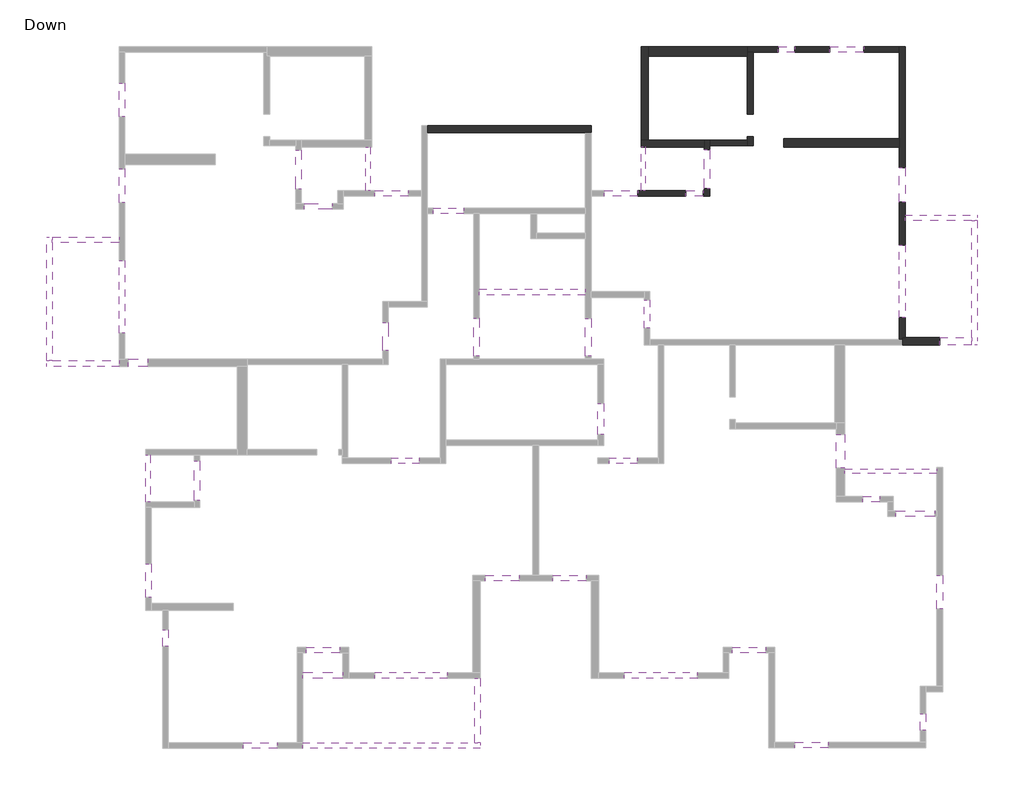
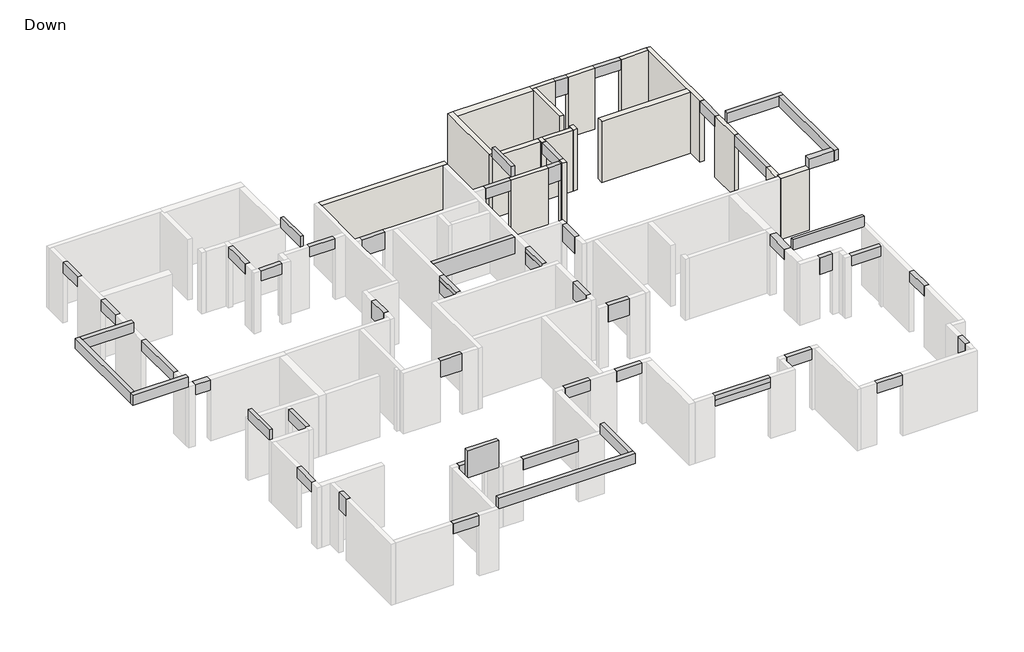
# One storey, part 3 of 3: 52 beams, 19 walls.
# Revit data of these elements (continued)
# Element 38 (IfcBeam, "Concrete Rectengular Beam : 20/82") (continued)
#   Phase Created = New Construction
#   Materials on its faces: "Concrete"
# Element 39 (IfcBeam, "Concrete Rectengular Beam : 20/82")
#   Comments = ""
#   Mark = "B42"
#   SOFiSTiK_AMG_Comments = ""
#   SOFiSTiK_AMG_Scheduled = yes
#   SOFiSTiK_AMG_Adjusted = yes
#   Structural Material = Concrete
#   Phase Created = New Construction
#   Materials on its faces: "Concrete"
# Element 40 (IfcBeam, "Concrete Rectengular Beam : 20/82")
#   Comments = ""
#   Mark = "B43"
#   SOFiSTiK_AMG_Comments = ""
#   SOFiSTiK_AMG_Scheduled = yes
#   SOFiSTiK_AMG_Adjusted = yes
#   Structural Material = Concrete
#   Phase Created = New Construction
#   Materials on its faces: "Concrete"
# Element 41 (IfcBeam, "Concrete Rectengular Beam : 20/82")
#   Comments = ""
#   Mark = "B44"
#   SOFiSTiK_AMG_Comments = ""
#   SOFiSTiK_AMG_Scheduled = yes
#   SOFiSTiK_AMG_Adjusted = yes
#   Structural Material = Concrete
#   Phase Created = New Construction
#   Materials on its faces: "Concrete"
# Element 42 (IfcBeam, "Concrete Rectengular Beam : 20/82")
#   Comments = ""
#   Mark = "B45"
#   SOFiSTiK_AMG_Comments = ""
#   SOFiSTiK_AMG_Scheduled = yes
#   SOFiSTiK_AMG_Adjusted = yes
#   Structural Material = Concrete
#   Phase Created = New Construction
#   Materials on its faces: "Concrete"
# Element 43 (IfcBeam, "Concrete Rectengular Beam : 20/82")
#   Comments = ""
#   Mark = "B46"
#   SOFiSTiK_AMG_Comments = ""
#   SOFiSTiK_AMG_Scheduled = yes
#   SOFiSTiK_AMG_Adjusted = yes
#   Structural Material = Concrete
#   Phase Created = New Construction
#   Materials on its faces: "Concrete"
# Element 44 (IfcBeam, "Concrete Rectengular Beam : 20/82")
#   Comments = ""
#   Mark = "B47"
#   SOFiSTiK_AMG_Comments = ""
#   SOFiSTiK_AMG_Scheduled = yes
#   SOFiSTiK_AMG_Adjusted = yes
#   Structural Material = Concrete
#   Phase Created = New Construction
#   Materials on its faces: "Concrete"
# Element 45 (IfcBeam, "Concrete Rectengular Beam : 20/82")
#   Comments = ""
#   Mark = "B48"
#   SOFiSTiK_AMG_Comments = ""
#   SOFiSTiK_AMG_Scheduled = yes
#   SOFiSTiK_AMG_Adjusted = yes
#   Structural Material = Concrete
#   Phase Created = New Construction
#   Materials on its faces: "Concrete"
# Element 46 (IfcBeam, "Concrete Rectengular Beam : 20/82")
#   Comments = ""
#   Mark = "B49"
#   SOFiSTiK_AMG_Comments = ""
#   SOFiSTiK_AMG_Scheduled = yes
#   SOFiSTiK_AMG_Adjusted = yes
#   Structural Material = Concrete
#   Phase Created = New Construction
#   Materials on its faces: "Concrete"
# Element 47 (IfcBeam, "Concrete Rectengular Beam : 20/82")
#   Comments = ""
#   Mark = "B50"
#   SOFiSTiK_AMG_Comments = ""
#   SOFiSTiK_AMG_Scheduled = yes
#   SOFiSTiK_AMG_Adjusted = yes
#   Structural Material = Concrete
#   Phase Created = New Construction
#   Materials on its faces: "Concrete"
# Element 48 (IfcBeam, "Concrete Rectengular Beam : 20/82")
#   Comments = ""
#   Mark = "B51"
#   SOFiSTiK_AMG_Comments = ""
#   SOFiSTiK_AMG_Scheduled = yes
#   SOFiSTiK_AMG_Adjusted = yes
#   Structural Material = Concrete
#   Phase Created = New Construction
#   Materials on its faces: "Concrete"
# Element 49 (IfcBeam, "Concrete Rectengular Beam : 20/82")
#   Comments = ""
#   Mark = "B52"
#   SOFiSTiK_AMG_Comments = ""
#   SOFiSTiK_AMG_Scheduled = yes
#   SOFiSTiK_AMG_Adjusted = yes
#   Structural Material = Concrete
#   Phase Created = New Construction
#   Materials on its faces: "Concrete"
# Element 50 (IfcBeam, "Concrete Rectengular Beam : 27/50")
#   Comments = ""
#   Mark = "B53"
#   SOFiSTiK_AMG_Comments = ""
#   SOFiSTiK_AMG_Scheduled = yes
#   SOFiSTiK_AMG_Adjusted = yes
#   Structural Material = Concrete
#   Phase Created = New Construction
#   Materials on its faces: "Concrete"
# Element 51 (IfcBeam, "Concrete Rectengular Beam : 27/50")
#   Comments = ""
#   Mark = "B54"
#   SOFiSTiK_AMG_Comments = ""
#   SOFiSTiK_AMG_Scheduled = yes
#   SOFiSTiK_AMG_Adjusted = yes
#   Structural Material = Concrete
#   Phase Created = New Construction
#   Materials on its faces: "Concrete"
# Element 52 (IfcBeam, "Concrete Rectengular Beam : 30/50")
#   Comments = ""
#   Mark = "B55"
#   SOFiSTiK_AMG_Comments = ""
#   SOFiSTiK_AMG_Scheduled = yes
#   SOFiSTiK_AMG_Adjusted = yes
#   Structural Material = Concrete
#   Phase Created = New Construction
#   Materials on its faces: "Concrete"
# Element 53 (IfcWall, "20")
#   Comments = ""
#   Mark = "W87"
#   SOFiSTiK_EdgeZones = "W87"
#   SOFiSTiK_AMG_Comments = ""
#   Top Offset = 0 cm
#   Base Offset = 0 cm
#   wall height = 300 cm
#   SOFiSTiK_AMG_Scheduled = yes
#   SOFiSTiK_AMG_Adjusted = yes
#   Phase Created = New Construction
#   Base Constraint = Down
#   Top Constraint = Typical Floor
#   Materials on its faces: "Concrete"
# Element 54 (IfcWall, "20")
#   Comments = ""
#   Mark = "W88"
#   SOFiSTiK_EdgeZones = "W88"
#   SOFiSTiK_AMG_Comments = ""
#   Top Offset = 0 cm
#   Base Offset = 0 cm
#   wall height = 300 cm
#   SOFiSTiK_AMG_Scheduled = yes
#   SOFiSTiK_AMG_Adjusted = yes
#   Phase Created = New Construction
#   Base Constraint = Down
#   Top Constraint = Typical Floor
#   Materials on its faces: "Concrete"
# Element 55 (IfcWall, "20")
#   Comments = ""
#   Mark = "W89"
#   SOFiSTiK_EdgeZones = "W89"
#   SOFiSTiK_AMG_Comments = ""
#   Top Offset = 0 cm
#   Base Offset = 0 cm
#   wall height = 300 cm
#   SOFiSTiK_AMG_Scheduled = yes
#   SOFiSTiK_AMG_Adjusted = yes
#   Phase Created = New Construction
#   Base Constraint = Down
#   Top Constraint = Typical Floor
#   Materials on its faces: "Concrete"
# Element 56 (IfcWall, "20")
#   Comments = ""
#   Mark = "W90"
#   SOFiSTiK_EdgeZones = "W90"
#   SOFiSTiK_AMG_Comments = ""
#   Top Offset = 0 cm
#   Base Offset = 0 cm
#   wall height = 300 cm
#   SOFiSTiK_AMG_Scheduled = yes
#   SOFiSTiK_AMG_Adjusted = yes
#   Phase Created = New Construction
#   Base Constraint = Down
#   Top Constraint = Typical Floor
#   Materials on its faces: "Concrete"
# Element 57 (IfcWall, "20")
#   Comments = ""
#   Mark = "W91"
#   SOFiSTiK_EdgeZones = "W91"
#   SOFiSTiK_AMG_Comments = ""
#   Top Offset = 0 cm
#   Base Offset = 0 cm
#   wall height = 300 cm
#   SOFiSTiK_AMG_Scheduled = yes
#   SOFiSTiK_AMG_Adjusted = yes
#   Phase Created = New Construction
#   Base Constraint = Down
#   Top Constraint = Typical Floor
#   Materials on its faces: "Concrete"
# Element 58 (IfcWall, "20")
#   Comments = ""
#   Mark = "W92"
#   SOFiSTiK_EdgeZones = "W92"
#   SOFiSTiK_AMG_Comments = ""
#   Top Offset = 0 cm
#   Base Offset = 0 cm
#   wall height = 300 cm
#   SOFiSTiK_AMG_Scheduled = yes
#   SOFiSTiK_AMG_Adjusted = yes
#   Phase Created = New Construction
#   Base Constraint = Down
#   Top Constraint = Typical Floor
#   Materials on its faces: "Concrete"
# Element 59 (IfcWall, "20")
#   Comments = ""
#   Mark = "W93"
#   SOFiSTiK_EdgeZones = "W93"
#   SOFiSTiK_AMG_Comments = ""
#   Top Offset = 0 cm
#   Base Offset = 0 cm
#   wall height = 300 cm
#   SOFiSTiK_AMG_Scheduled = yes
#   SOFiSTiK_AMG_Adjusted = yes
#   Phase Created = New Construction
#   Base Constraint = Down
#   Top Constraint = Typical Floor
#   Materials on its faces: "Concrete"
# Element 60 (IfcWall, "20")
#   Comments = ""
#   Mark = "W94"
#   SOFiSTiK_EdgeZones = "W94"
#   SOFiSTiK_AMG_Comments = ""
#   Top Offset = 0 cm
#   Base Offset = 0 cm
#   wall height = 300 cm
#   SOFiSTiK_AMG_Scheduled = yes
#   SOFiSTiK_AMG_Adjusted = yes
#   Phase Created = New Construction
#   Base Constraint = Down
#   Top Constraint = Typical Floor
#   Materials on its faces: "Concrete"
# Element 61 (IfcWall, "20")
#   Comments = ""
#   Mark = "W95"
#   SOFiSTiK_EdgeZones = "W95"
#   SOFiSTiK_AMG_Comments = ""
#   Top Offset = 0 cm
#   Base Offset = 0 cm
#   wall height = 300 cm
#   SOFiSTiK_AMG_Scheduled = yes
#   SOFiSTiK_AMG_Adjusted = yes
#   Phase Created = New Construction
#   Base Constraint = Down
#   Top Constraint = Typical Floor
#   Materials on its faces: "Concrete"
# Element 62 (IfcWall, "20")
#   Comments = ""
#   Mark = "W96"
#   SOFiSTiK_EdgeZones = "W96"
#   SOFiSTiK_AMG_Comments = ""
#   Top Offset = 0 cm
#   Base Offset = 0 cm
#   wall height = 300 cm
#   SOFiSTiK_AMG_Scheduled = yes
#   SOFiSTiK_AMG_Adjusted = yes
#   Phase Created = New Construction
#   Base Constraint = Down
#   Top Constraint = Typical Floor
#   Materials on its faces: "Concrete"
# Element 63 (IfcWall, "20")
#   Comments = ""
#   Mark = "W97"
#   SOFiSTiK_EdgeZones = "W97"
#   SOFiSTiK_AMG_Comments = ""
#   Top Offset = 0 cm
#   Base Offset = 0 cm
#   wall height = 300 cm
#   SOFiSTiK_AMG_Scheduled = yes
#   SOFiSTiK_AMG_Adjusted = yes
#   Phase Created = New Construction
#   Base Constraint = Down
#   Top Constraint = Typical Floor
#   Materials on its faces: "Concrete"
# Element 64 (IfcWall, "20")
#   Comments = ""
#   Mark = "W98"
#   SOFiSTiK_EdgeZones = "W98"
#   SOFiSTiK_AMG_Comments = "Too Short /"
#   Top Offset = 0 cm
#   Base Offset = 0 cm
#   wall height = 300 cm
#   SOFiSTiK_AMG_Scheduled = yes
#   SOFiSTiK_AMG_Adjusted = yes
#   Phase Created = New Construction
#   Base Constraint = Down
#   Top Constraint = Typical Floor
#   Materials on its faces: "Concrete"
# Element 65 (IfcWall, "20")
#   Comments = ""
#   Mark = "W99"
#   SOFiSTiK_EdgeZones = "W99"
#   SOFiSTiK_AMG_Comments = ""
#   Top Offset = 0 cm
#   Base Offset = 0 cm
#   wall height = 300 cm
#   SOFiSTiK_AMG_Scheduled = yes
#   SOFiSTiK_AMG_Adjusted = yes
#   Phase Created = New Construction
#   Base Constraint = Down
#   Top Constraint = Typical Floor
#   Materials on its faces: "Concrete"
# Element 66 (IfcWall, "25")
#   Comments = ""
#   Mark = "W115"
#   SOFiSTiK_EdgeZones = "W115"
#   SOFiSTiK_AMG_Comments = ""
#   Top Offset = 0 cm
#   Base Offset = 0 cm
#   wall height = 300 cm
#   SOFiSTiK_AMG_Scheduled = yes
#   SOFiSTiK_AMG_Adjusted = yes
#   Phase Created = New Construction
#   Base Constraint = Down
#   Top Constraint = Typical Floor
#   Materials on its faces: "Concrete"
# Element 67 (IfcWall, "25")
#   Comments = ""
#   Mark = "W117"
#   SOFiSTiK_EdgeZones = "W117"
#   SOFiSTiK_AMG_Comments = ""
#   Top Offset = 0 cm
#   Base Offset = 0 cm
#   wall height = 300 cm
#   SOFiSTiK_AMG_Scheduled = yes
#   SOFiSTiK_AMG_Adjusted = yes
#   Phase Created = New Construction
#   Base Constraint = Down
#   Top Constraint = Typical Floor
#   Materials on its faces: "Concrete"
# Element 68 (IfcWall, "25")
#   Comments = ""
#   Mark = "W118"
#   SOFiSTiK_EdgeZones = "W118"
#   SOFiSTiK_AMG_Comments = ""
#   Top Offset = 0 cm
#   Base Offset = 0 cm
#   wall height = 300 cm
#   SOFiSTiK_AMG_Scheduled = yes
#   SOFiSTiK_AMG_Adjusted = yes
#   Phase Created = New Construction
#   Base Constraint = Down
#   Top Constraint = Typical Floor
#   Materials on its faces: "Concrete"
# Element 69 (IfcWall, "27")
#   Comments = ""
#   Mark = "W112"
#   SOFiSTiK_EdgeZones = "W112"
#   SOFiSTiK_AMG_Comments = ""
#   Top Offset = 0 cm
#   Base Offset = 0 cm
#   wall height = 300 cm
#   SOFiSTiK_AMG_Scheduled = yes
#   SOFiSTiK_AMG_Adjusted = yes
#   Phase Created = New Construction
#   Base Constraint = Down
#   Top Constraint = Typical Floor
#   Materials on its faces: "Concrete"
# Element 70 (IfcWall, "30")
#   Comments = ""
#   Mark = "W122"
#   SOFiSTiK_EdgeZones = "W122"
#   SOFiSTiK_AMG_Comments = ""
#   Top Offset = 0 cm
#   Base Offset = 0 cm
#   wall height = 300 cm
#   SOFiSTiK_AMG_Scheduled = yes
#   SOFiSTiK_AMG_Adjusted = yes
#   Phase Created = New Construction
#   Base Constraint = Down
#   Top Constraint = Typical Floor
#   Materials on its faces: "Concrete"
# Element 71 (IfcWall, "35")
#   Comments = ""
#   Mark = "W3"
#   SOFiSTiK_EdgeZones = "W3"
#   SOFiSTiK_AMG_Comments = ""
#   Top Offset = 0 cm
#   Base Offset = 0 cm
#   wall height = 300 cm
#   SOFiSTiK_AMG_Scheduled = yes
#   SOFiSTiK_AMG_Adjusted = yes
#   Phase Created = New Construction
#   Base Constraint = Down
#   Top Constraint = Typical Floor
#   Materials on its faces: "Concrete"
# Materials
#   "Concrete": class "Concrete", colour RGB 192 192 192, transparency 0, Keynote = "01000", Description = "Cast-in-place concrete", Cost = 0
